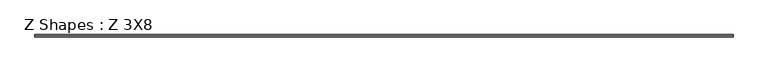
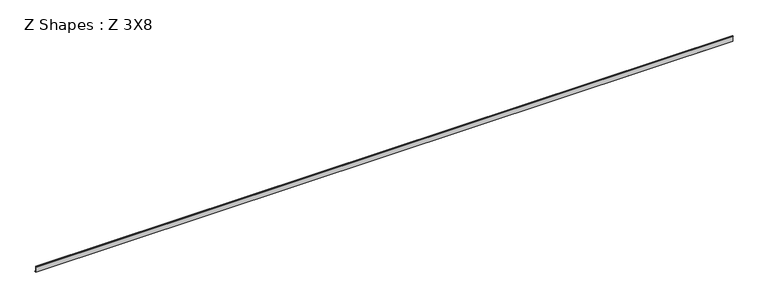
"""IFC4 building model written with IfcOpenShell, lengths in millimetres: beam geometry, Z Shapes : Z 3X8."""

from ifc_helpers import new_model, si_unit, frame, origin, place, context, project, spatial, polyline, outline, extrude, source, transform, mapped, element, save


def z_shapes_z_3x8_8fd8e94e(model_context):
    return source(origin(), model_context, "Body", "SweptSolid", [
        extrude(outline(polyline([(-57.2805719, 92.452825), (-57.2805719, 102.104825), (-19.1805719, 102.104825), (-19.1805719, -92.459175), (18.9194281, -92.459175), (18.9194281, -98.809175), (-27.1991352, -98.809175), (-27.1991352, 92.452825), (-57.2805719, 92.452825)])), frame((-11671.3, 0.0, 0.0), z_axis=(1.0, 0.0, 0.0), x_axis=(0.0, 1.0, 0.0)), (0.0, 0.0, 1.0), 23342.6),
    ])


if __name__ == "__main__":
    model = new_model("IFC4")
    model_context = context("Model", 3, world=origin())
    ifc_project = project(units=[si_unit("LENGTHUNIT", "METRE", prefix="MILLI")], contexts=[model_context])
    site = spatial("IfcSite", under=ifc_project)
    building = spatial("IfcBuilding", under=site)
    placement = place(None, origin())
    z_shapes_z_3x8_shape = z_shapes_z_3x8_8fd8e94e(model_context)
    element("IfcBeam", 1, ObjectType="Z Shapes : Z 3X8", at=placement, inside=building, context=model_context, shape_type="MappedRepresentation", body=[
        mapped(z_shapes_z_3x8_shape, transform((0.0, 0.0, 0.0), x_axis=(1.0, 0.0, 0.0), y_axis=(0.0, 1.0, 0.0), z_axis=(0.0, 0.0, 1.0))),
    ])
    save(model, "model.ifc")

# Revit data of these elements
# Type "Z Shapes : Z 3X8"
#   Section Name Key = "W12x26"
#   Assembly Code = "B10"
#   Width = 76.2 mm
#   Web Thickness = 5.842 mm
#   Web Fillet = 7.62 mm
#   Warping Constant = 163001.3 cm⁶
#   Torsional Moment of Inertia = 12.4869 cm⁴
#   Section Area = 7.65 in²
#   Plastic Modulus weak axis = 0.00472801 (stored number, unit not read)
#   Plastic Modulus strong axis = 0.0215278 (stored number, unit not read)
#   Perimeter = 15.0571 m²/m
#   Nominal Weight = 379.441 N/m
#   Moment of Inertia weak axis = 720.08 cm⁴
#   Moment of Inertia strong axis = 8491.12 cm⁴
#   Height = 184.912 mm
#   Flange Thickness = 9.652 mm
#   Elastic Modulus weak axis = 0.00309028 (stored number, unit not read)
#   Elastic Modulus strong axis = 0.0193287 (stored number, unit not read)
#   Centroid Vertical = 92.456 mm
#   Centroid Horizontal = 38.1 mm
#   Length [instance default] = 5' - 0"
#   Structural Material [instance default] = Steel ASTM A992
#   Principal Axes Angle = 0
# Element 1 (IfcBeam, "Z Shapes : Z 3X8")
#   Structural Material = accent 2
#   Materials on its faces: "accent 2"
# Materials
#   "Steel ASTM A992": class "Metal", colour RGB 189 187 185, transparency 0, Description = "Structural steel 50ksi", Cost = 0
#   "accent 2": class "Wood", colour RGB 80 80 80, transparency 0, Description = "Wood framing, thermal airspace", Cost = 0
